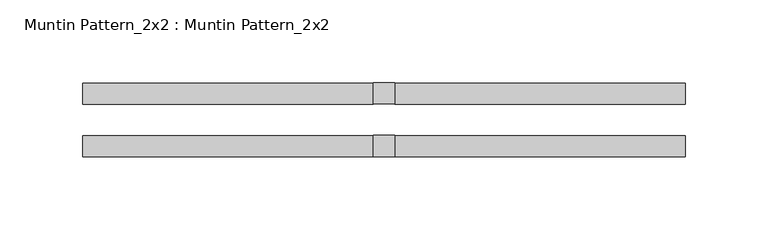
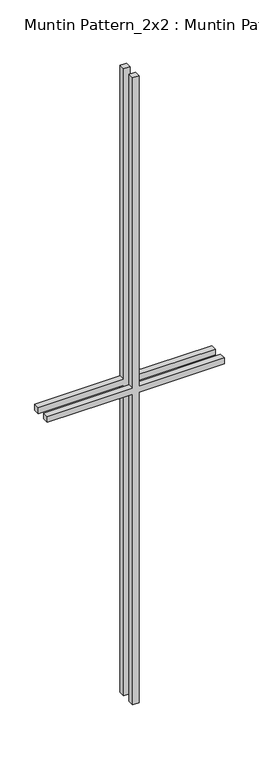
"""IFC4 building model written with IfcOpenShell, lengths in millimetres: proxy geometry, Muntin Pattern_2x2 : Muntin Pattern_2x2."""

import ifcopenshell
import ifcopenshell.guid

model = None  # the IFC model being written
_history = None  # IfcOwnerHistory: only IFC2X3 demands one
_inside = {}  # id of a spatial element -> (the spatial element, [elements in it])
_under = {}  # id of a project, library or spatial element -> (it, [spatial elements below it])
_declared = {}  # id of a project -> (the project, [libraries it declares])
_typed = {}  # id of a type object -> (the type object, [elements of that type])
_made_of = {}  # id of a material, layer set ... -> (it, [elements and type objects made of it])


def new_model(schema):
    """Start an empty IFC model of exactly this schema.

    Asked for "IFC4X3", IfcOpenShell would pick the latest addendum, in which some entities
    have other attributes; the version numbers below select the first issue.
    IFC2X3 requires an IfcOwnerHistory on every rooted entity: one is made here for all.
    """
    global model, _history
    if schema == "IFC4X3":
        model = ifcopenshell.file(schema_version=(4, 3, 0, 0))
    else:
        model = ifcopenshell.file(schema=schema)
    _inside.clear()
    _under.clear()
    _declared.clear()
    _typed.clear()
    _made_of.clear()
    _history = None
    if model.schema == "IFC2X3":
        org = make("IfcOrganization", Name="unknown")
        user = make(
            "IfcPersonAndOrganization",
            ThePerson=make("IfcPerson", FamilyName="unknown"),
            TheOrganization=org,
        )
        app = make(
            "IfcApplication",
            ApplicationDeveloper=org,
            Version="unknown",
            ApplicationFullName="unknown",
            ApplicationIdentifier="unknown",
        )
        _history = make(
            "IfcOwnerHistory",
            OwningUser=user,
            OwningApplication=app,
            ChangeAction="ADDED",
            CreationDate=0,
        )
    return model


def make(cls, **values):
    """One entity of the class cls with the attributes given. An attribute that is None is left unset."""
    return model.create_entity(
        cls, **{name: value for name, value in values.items() if value is not None}
    )


def rooted(cls, **values):
    """An entity with a GlobalId (a new one), such as an element, a storey or a relation."""
    return make(cls, GlobalId=ifcopenshell.guid.new(), OwnerHistory=_history, **values)


def si_unit(unit_type, name, prefix=None):
    """IfcSIUnit, for example si_unit("LENGTHUNIT", "METRE", prefix="MILLI")."""
    return make("IfcSIUnit", UnitType=unit_type, Prefix=prefix, Name=name)


def assignment(units):
    """IfcUnitAssignment: the units of a project."""
    return None if units is None else make("IfcUnitAssignment", Units=units)


def point(xyz):
    """IfcCartesianPoint."""
    return None if xyz is None else make("IfcCartesianPoint", Coordinates=xyz)


def direction(xyz):
    """IfcDirection."""
    return None if xyz is None else make("IfcDirection", DirectionRatios=xyz)


def frame(location, z_axis=None, x_axis=None):
    """IfcAxis2Placement3D, a coordinate frame: its origin and axes. An axis left out is left unset."""
    return make(
        "IfcAxis2Placement3D",
        Location=point(location),
        Axis=direction(z_axis),
        RefDirection=direction(x_axis),
    )


def origin():
    """The frame at (0, 0, 0) with its axes left unset."""
    return frame((0.0, 0.0, 0.0))


def place(relative_to, where):
    """IfcLocalPlacement: puts the frame where relative to a parent placement (None: the world)."""
    return make(
        "IfcLocalPlacement", PlacementRelTo=relative_to, RelativePlacement=where
    )


def context(
    kind, dimensions, precision=None, world=None, true_north=None, identifier=None
):
    """IfcGeometricRepresentationContext, for example the 3D "Model" context."""
    return make(
        "IfcGeometricRepresentationContext",
        ContextIdentifier=identifier,
        ContextType=kind,
        CoordinateSpaceDimension=dimensions,
        Precision=precision,
        WorldCoordinateSystem=world,
        TrueNorth=true_north,
    )


def project(units=None, contexts=None):
    """IfcProject with its units and contexts."""
    return rooted(
        "IfcProject",
        Name="project",
        RepresentationContexts=contexts,
        UnitsInContext=assignment(units),
    )


def spatial(cls, under=None, at=None, **own):
    """A site, building, storey or space (cls), placed at a placement, below another one or the project."""
    s = rooted(cls, ObjectPlacement=at, **own)
    if under is not None:
        _under.setdefault(under.id(), (under, []))[1].append(s)
    return s


def polyline(points):
    """IfcPolyline through the points."""
    return make("IfcPolyline", Points=[point(p) for p in points])


def outline(outer, holes=None, kind="AREA"):
    """IfcArbitraryClosedProfileDef: a profile drawn as a closed curve; with holes, ...WithVoids."""
    if holes is None:
        return make("IfcArbitraryClosedProfileDef", ProfileType=kind, OuterCurve=outer)
    return make(
        "IfcArbitraryProfileDefWithVoids",
        ProfileType=kind,
        OuterCurve=outer,
        InnerCurves=holes,
    )


def extrude(swept, where, along, depth):
    """IfcExtrudedAreaSolid: the profile swept, set in the frame where, extruded along a direction by depth."""
    return make(
        "IfcExtrudedAreaSolid",
        SweptArea=swept,
        Position=where,
        ExtrudedDirection=direction(along),
        Depth=depth,
    )


def shape(context_of_items, identifier, shape_type, items):
    """IfcShapeRepresentation: the items that make up one representation, for example the "Body"."""
    return make(
        "IfcShapeRepresentation",
        ContextOfItems=context_of_items,
        RepresentationIdentifier=identifier,
        RepresentationType=shape_type,
        Items=items,
    )


def source(mapping_origin, context_of_items, identifier, shape_type, items):
    """IfcRepresentationMap: a shape defined once, which mapped items show again and again."""
    return make(
        "IfcRepresentationMap",
        MappingOrigin=mapping_origin,
        MappedRepresentation=shape(context_of_items, identifier, shape_type, items),
    )


def transform(
    local_origin,
    x_axis=None,
    y_axis=None,
    z_axis=None,
    scale=None,
    scale2=None,
    scale3=None,
    uniform=True,
):
    """IfcCartesianTransformationOperator3D, or its non-uniform kind. x_axis, y_axis, z_axis: its Axis1, 2, 3."""
    if uniform:
        return make(
            "IfcCartesianTransformationOperator3D",
            Axis1=direction(x_axis),
            Axis2=direction(y_axis),
            LocalOrigin=point(local_origin),
            Scale=scale,
            Axis3=direction(z_axis),
        )
    return make(
        "IfcCartesianTransformationOperator3DnonUniform",
        Axis1=direction(x_axis),
        Axis2=direction(y_axis),
        LocalOrigin=point(local_origin),
        Scale=scale,
        Axis3=direction(z_axis),
        Scale2=scale2,
        Scale3=scale3,
    )


def mapped(mapping_source, mapping_target):
    """IfcMappedItem: shows the shape of a source again, moved by a transform."""
    return make(
        "IfcMappedItem", MappingSource=mapping_source, MappingTarget=mapping_target
    )


def made_of(thing, what):
    """Note that an element or type object is made of a material, layer set ...; save() writes the relation."""
    if what is not None:
        _made_of.setdefault(what.id(), (what, []))[1].append(thing)
    return thing


def element(
    cls,
    number,
    at=None,
    inside=None,
    cuts=None,
    type_object=None,
    material=None,
    context=None,
    identifier="Body",
    shape_type=None,
    held_by="IfcProductDefinitionShape",
    body=None,
    shapes=None,
    **own,
):
    """One element of the class cls, such as IfcWall. Its Tag is "e" and its number.

    at: its placement. inside: the storey or other place that contains it. cuts: it is an
    opening in that element (IfcRelVoidsElement). A single representation is given by context,
    identifier, shape_type and body (its items); several are given by shapes. held_by: the class
    of the entity that holds the representations. save() writes the other relations.
    """
    e = rooted(cls, Tag="e%d" % number, ObjectPlacement=at, **own)
    if body is not None:
        shapes = [shape(context, identifier, shape_type, body)]
    if shapes is not None:
        e.Representation = make(held_by, Representations=shapes)
    if inside is not None:
        _inside.setdefault(inside.id(), (inside, []))[1].append(e)
    if cuts is not None:
        rooted(
            "IfcRelVoidsElement", RelatingBuildingElement=cuts, RelatedOpeningElement=e
        )
    if type_object is not None:
        _typed.setdefault(type_object.id(), (type_object, []))[1].append(e)
    return made_of(e, material)


def aggregate(whole, parts):
    """IfcRelAggregates: a whole, such as a stair, and the parts it consists of."""
    return rooted("IfcRelAggregates", RelatingObject=whole, RelatedObjects=parts)


def save(model, path):
    """Write the relations noted so far, then the file.

    IfcRelAggregates (storeys below a building ...), IfcRelContainedInSpatialStructure (elements
    in a storey), IfcRelDefinesByType, IfcRelAssociatesMaterial and IfcRelDeclares: one each for
    every whole, place, type object, material and project.
    """
    for whole, parts in _under.values():
        aggregate(whole, parts)
    for where, things in _inside.values():
        rooted(
            "IfcRelContainedInSpatialStructure",
            RelatedElements=things,
            RelatingStructure=where,
        )
    for kind, things in _typed.values():
        rooted("IfcRelDefinesByType", RelatedObjects=things, RelatingType=kind)
    for what, things in _made_of.values():
        rooted("IfcRelAssociatesMaterial", RelatedObjects=things, RelatingMaterial=what)
    for by, libraries in _declared.values():
        rooted("IfcRelDeclares", RelatingContext=by, RelatedDefinitions=libraries)
    model.write(path)


def muntin_pattern_2x2_muntin_pattern_2x2_cbb9fd28(model_context):
    return source(origin(), model_context, "Body", "SweptSolid", [
        extrude(outline(polyline([(686.5, -6.35), (686.5, -181.7375), (673.8, -181.7375), (673.8, -6.35), (0.0, -6.35), (0.0, 6.35), (673.8, 6.35), (673.8, 181.7375), (686.5, 181.7375), (686.5, 6.35), (1360.3, 6.35), (1360.3, -6.35), (686.5, -6.35)])), frame((0.0, 9.525, 0.0), z_axis=(0.0, 1.0, 0.0), x_axis=(0.0, 0.0, 1.0)), (0.0, 0.0, 1.0), 12.7),
        extrude(outline(polyline([(686.5, -6.35), (686.5, -181.7375), (673.8, -181.7375), (673.8, -6.35), (0.0, -6.35), (0.0, 6.35), (673.8, 6.35), (673.8, 181.7375), (686.5, 181.7375), (686.5, 6.35), (1360.3, 6.35), (1360.3, -6.35), (686.5, -6.35)])), frame((0.0, -22.225, 0.0), z_axis=(0.0, 1.0, 0.0), x_axis=(0.0, 0.0, 1.0)), (0.0, 0.0, 1.0), 12.7),
    ])


if __name__ == "__main__":
    model = new_model("IFC4")
    model_context = context("Model", 3, world=origin())
    ifc_project = project(units=[si_unit("LENGTHUNIT", "METRE", prefix="MILLI")], contexts=[model_context])
    site = spatial("IfcSite", under=ifc_project)
    building = spatial("IfcBuilding", under=site)
    placement = place(None, origin())
    muntin_pattern_2x2_muntin_pattern_2x2_shape = muntin_pattern_2x2_muntin_pattern_2x2_cbb9fd28(model_context)
    element("IfcBuildingElementProxy", 1, Name="Muntin Pattern_2x2 : Muntin Pattern_2x2", ObjectType="Muntin Pattern_2x2 : Muntin Pattern_2x2", at=placement, inside=building, context=model_context, shape_type="MappedRepresentation", body=[
        mapped(muntin_pattern_2x2_muntin_pattern_2x2_shape, transform((0.0, 0.0, 0.0), x_axis=(1.0, 0.0, 0.0), y_axis=(0.0, 1.0, 0.0), z_axis=(0.0, 0.0, 1.0))),
    ])
    save(model, "model.ifc")

# Revit data of these elements
# Type "Muntin Pattern_2x2 : Muntin Pattern_2x2"
#   Width [instance default] = 1.2192 m
#   Thickness = 0.0127 m
#   Height [instance default] = 1.2192 m
#   Distance = 0.01905 m
#   Interior Material [instance default] = none
#   Exterior Material [instance default] = none
# Element 1 (IfcBuildingElementProxy, "Muntin Pattern_2x2 : Muntin Pattern_2x2")
#   Width = 0.363475 m
#   Height = 1.3603 m
#   Interior Material = Wood - Stained
#   Exterior Material = Clad - White
#   Materials on its faces: "Clad - White", "Wood - Stained"
# Materials
#   "Clad - White": class "Wood", colour RGB 242 242 238, transparency 0, Cost = 0
#   "Wood - Stained": class "Wood", colour RGB 224 178 126, transparency 0, Cost = 0
